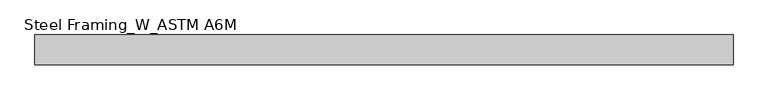
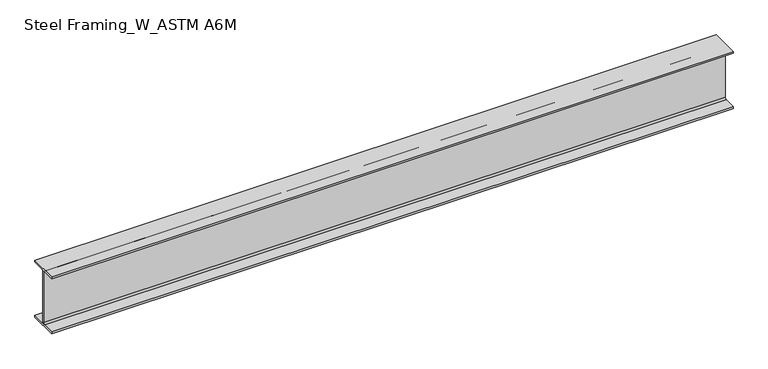
"""IFC4 building model written with IfcOpenShell, lengths in millimetres: beam geometry, Steel Framing_W_ASTM A6M : H_SB_AR_S02_W360x51_RG1."""

from ifc_helpers import new_model, si_unit, point, frame, frame_2d, origin, place, context, project, spatial, polyline, circle_curve, trimmed, segment, composite_curve, outline, extrude, source, transform, mapped, element, save


def steel_framing_w_astm_a6m_8f8296d1(model_context):
    return source(origin(), model_context, "Body", "SweptSolid", [
        extrude(outline(composite_curve([segment(polyline([(85.5, -166.4), (85.5, -178.0), (-85.5, -178.0), (-85.5, -166.4), (-13.72, -166.4)]), True, "CONTINUOUS"), segment(trimmed(circle_curve(frame_2d((-13.72, -156.3)), 10.1), [point((-13.72, -166.4))], [point((-3.62, -156.3))], True, "CARTESIAN"), True, "CONTINUOUS"), segment(polyline([(-3.62, -156.3), (-3.62, 156.3)]), True, "CONTINUOUS"), segment(trimmed(circle_curve(frame_2d((-13.72, 156.3)), 10.1), [point((-3.62, 156.3))], [point((-13.72, 166.4))], True, "CARTESIAN"), True, "CONTINUOUS"), segment(polyline([(-13.72, 166.4), (-85.5, 166.4), (-85.5, 178.0), (85.5, 178.0), (85.5, 166.4), (13.72, 166.4)]), True, "CONTINUOUS"), segment(trimmed(circle_curve(frame_2d((13.72, 156.3)), 10.1), [point((13.72, 166.4))], [point((3.62, 156.3))], True, "CARTESIAN"), True, "CONTINUOUS"), segment(polyline([(3.62, 156.3), (3.62, -156.3)]), True, "CONTINUOUS"), segment(trimmed(circle_curve(frame_2d((13.72, -156.3)), 10.1), [point((3.62, -156.3))], [point((13.72, -166.4))], True, "CARTESIAN"), True, "CONTINUOUS"), segment(polyline([(13.72, -166.4), (85.5, -166.4)]), True, "CONTINUOUS")], self_intersect=False)), frame((-2008.8, 0.0, 0.0), z_axis=(1.0, 0.0, 0.0), x_axis=(0.0, 1.0, 0.0)), (0.0, 0.0, 1.0), 4017.6),
    ])


if __name__ == "__main__":
    model = new_model("IFC4")
    model_context = context("Model", 3, world=origin())
    ifc_project = project(units=[si_unit("LENGTHUNIT", "METRE", prefix="MILLI")], contexts=[model_context])
    site = spatial("IfcSite", under=ifc_project)
    building = spatial("IfcBuilding", under=site)
    placement = place(None, origin())
    steel_framing_w_astm_a6m_shape = steel_framing_w_astm_a6m_8f8296d1(model_context)
    element("IfcBeam", 1, ObjectType="Steel Framing_W_ASTM A6M : H_SB_AR_S02_W360x51_RG1", at=placement, inside=building, context=model_context, shape_type="MappedRepresentation", body=[
        mapped(steel_framing_w_astm_a6m_shape, transform((0.0, 0.0, 0.0), x_axis=(1.0, 0.0, 0.0), y_axis=(0.0, 1.0, 0.0), z_axis=(0.0, 0.0, 1.0))),
    ])
    save(model, "model.ifc")

# Revit data of these elements
# Type "Steel Framing_W_ASTM A6M : H_SB_AR_S02_W360x51_RG1"
#   Type Mark = "RG1"
#   Section Name Key = "W14x34"
#   Width = 17.1 cm
#   Web Thickness = 0.724 cm
#   Web Fillet = 1.01 cm
#   Warping Constant = 287000.0 cm⁶
#   Torsional Moment of Inertia = 23.70 cm⁴
#   Section Area = 64.5 cm²
#   Plastic Modulus weak axis = 174.0 cm³
#   Plastic Modulus strong axis = 895.0 cm³
#   Perimeter = 1.36 m²/m
#   Nominal Weight = 51.00 kgf/m
#   Moment of Inertia weak axis = 970.00 cm⁴
#   Moment of Inertia strong axis = 14200.00 cm⁴
#   Height = 35.6 cm
#   Flange Thickness = 1.16 cm
#   Elastic Modulus weak axis = 113.0 cm³
#   Elastic Modulus strong axis = 796.0 cm³
#   Centroid Vertical = 17.8 cm
#   Centroid Horizontal = 8.55 cm
#   Length [instance default] = 1500 mm
#   Structural Material [instance default] = Steel, 45-345
#   Bolt Spacing = 0
#   Assembly Code = ""
# Element 1 (IfcBeam, "Steel Framing_W_ASTM A6M : H_SB_AR_S02_W360x51_RG1")
#   Materials on its faces: "Steel, 45-345"
# Materials
#   "Steel, 45-345": class "Metal", colour RGB 189 187 185, transparency 0, Description = "Steel 345 MPa", Cost = 0
